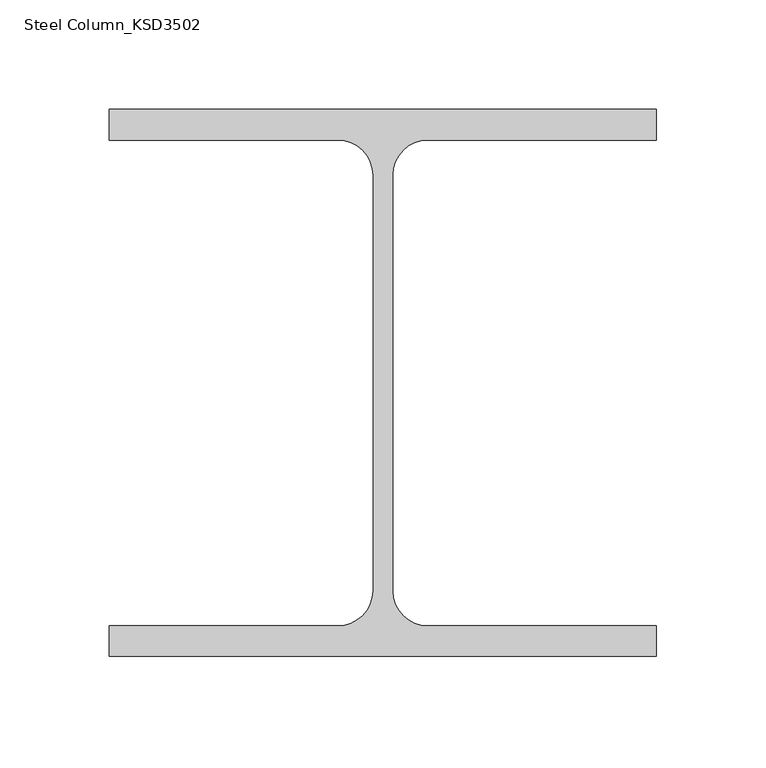
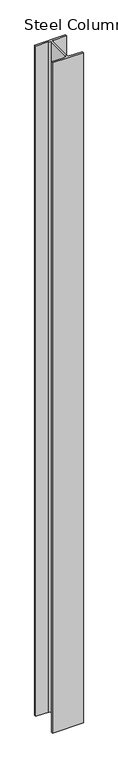
"""IFC4 building model written with IfcOpenShell, lengths in millimetres: column geometry, Steel Column_KSD3502 : H_SC_ASC_H-250×250x9x14."""

from ifc_helpers import new_model, si_unit, point, frame, frame_2d, origin, place, context, project, spatial, polyline, circle_curve, trimmed, segment, composite_curve, outline, extrude, source, transform, mapped, element, save


def steel_column_ksd3502_c27b98d8(model_context):
    return source(origin(), model_context, "Body", "SweptSolid", [
        extrude(outline(composite_curve([segment(polyline([(125.0, 125.0), (125.0, 111.0), (20.5, 111.0)]), True, "CONTINUOUS"), segment(trimmed(circle_curve(frame_2d((20.5, 95.0)), 16.0), [point((20.5, 111.0))], [point((4.5, 95.0))], True, "CARTESIAN"), True, "CONTINUOUS"), segment(polyline([(4.5, 95.0), (4.5, -95.0)]), True, "CONTINUOUS"), segment(trimmed(circle_curve(frame_2d((20.5, -95.0)), 16.0), [point((4.5, -95.0))], [point((20.5, -111.0))], True, "CARTESIAN"), True, "CONTINUOUS"), segment(polyline([(20.5, -111.0), (125.0, -111.0), (125.0, -125.0), (-125.0, -125.0), (-125.0, -111.0), (-20.5, -111.0)]), True, "CONTINUOUS"), segment(trimmed(circle_curve(frame_2d((-20.5, -95.0)), 16.0), [point((-20.5, -111.0))], [point((-4.5, -95.0))], True, "CARTESIAN"), True, "CONTINUOUS"), segment(polyline([(-4.5, -95.0), (-4.5, 95.0)]), True, "CONTINUOUS"), segment(trimmed(circle_curve(frame_2d((-20.5, 95.0)), 16.0), [point((-4.5, 95.0))], [point((-20.5, 111.0))], True, "CARTESIAN"), True, "CONTINUOUS"), segment(polyline([(-20.5, 111.0), (-125.0, 111.0), (-125.0, 125.0), (125.0, 125.0)]), True, "CONTINUOUS")], self_intersect=False)), frame((0.0, 0.0, 599.9720055), z_axis=(0.0, 0.0, 1.0), x_axis=(1.0, 0.0, 0.0)), (0.0, 0.0, 1.0), 5750.0),
    ])


if __name__ == "__main__":
    model = new_model("IFC4")
    model_context = context("Model", 3, world=origin())
    ifc_project = project(units=[si_unit("LENGTHUNIT", "METRE", prefix="MILLI")], contexts=[model_context])
    site = spatial("IfcSite", under=ifc_project)
    building = spatial("IfcBuilding", under=site)
    placement = place(None, origin())
    steel_column_ksd3502_shape = steel_column_ksd3502_c27b98d8(model_context)
    element("IfcColumn", 1, ObjectType="Steel Column_KSD3502 : H_SC_ASC_H-250×250x9x14", at=placement, inside=building, context=model_context, shape_type="MappedRepresentation", body=[
        mapped(steel_column_ksd3502_shape, transform((0.0, 0.0, 0.0), x_axis=(1.0, 0.0, 0.0), y_axis=(0.0, 1.0, 0.0), z_axis=(0.0, 0.0, 1.0))),
    ])
    save(model, "model.ifc")

# Revit data of these elements
# Type "Steel Column_KSD3502 : H_SC_ASC_H-250×250x9x14"
#   Width = 25.0 cm
#   Web Thickness = 0.9 cm
#   Web Fillet = 1.6 cm
#   Warping Constant = 507646.0 cm⁶
#   Torsional Moment of Inertia = 51.4681 cm⁴
#   Section Area = 92.18 cm²
#   Plastic Modulus weak axis = 444.0 cm³
#   Plastic Modulus strong axis = 960.0 cm³
#   Perimeter = 1.27 m²/m
#   Nominal Weight = 72.40 kgf/m
#   Moment of Inertia weak axis = 3650.00 cm⁴
#   Moment of Inertia strong axis = 10800.00 cm⁴
#   Height = 25.0 cm
#   Flange Thickness = 1.4 cm
#   Elastic Modulus weak axis = 292.0 cm³
#   Elastic Modulus strong axis = 867.0 cm³
#   Centroid Vertical = 12.5 cm
#   Centroid Horizontal = 12.5 cm
#   Bolt Spacing = 13.97 cm
#   Structural Material [instance default] = Steel, 45-345
#   Section Name Key = ""
#   Assembly Code = ""
# Element 1 (IfcColumn, "Steel Column_KSD3502 : H_SC_ASC_H-250×250x9x14")
#   Structural Material = A03AD029-00005_Anchor Bolt (Installation only)_M24
#   Materials on its faces: "A03AD029-00005_Anchor Bolt (Installation only)_M24"
# Materials
#   "Steel, 45-345": class "Metal", colour RGB 189 187 185, transparency 0, Description = "Steel 345 MPa", Cost = 0
#   "A03AD029-00005_Anchor Bolt (Installation only)_M24": class "Unassigned", colour RGB 84 83 81, transparency 0, Cost = 0
